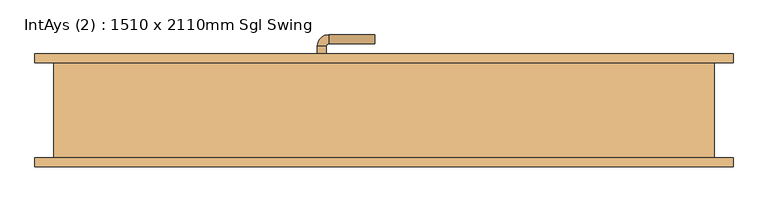
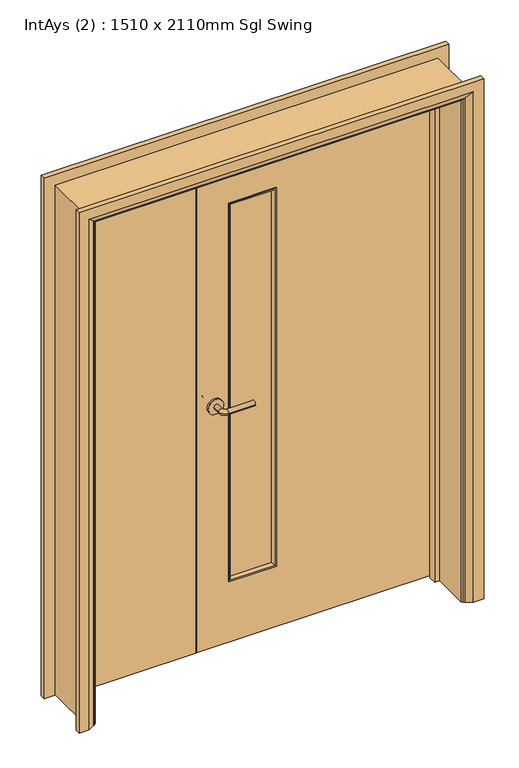
"""IFC4 building model written with IfcOpenShell, lengths in millimetres: door geometry, IntAys (2) : 1510 x 2110mm Sgl Swing."""

from ifc_helpers import new_model, si_unit, point, frame, frame_2d, origin, place, context, project, spatial, polyline, circle_curve, ellipse_curve, trimmed, segment, composite_curve, outline, extrude, faceted_brep, source, transform, mapped, element, save
from ifc_brep_helpers import plane_surface, cylinder_surface, revolved_surface, advanced_brep


def intays_2_1510_x_2110mm_sgl_swing_d010f506(model_context):
    return source(origin(), model_context, "Body", "SolidModel", [
        advanced_brep(
        [(88.5, 67.5, 1000.0), (108.5, 67.5, 1000.0), (108.5, 37.5, 1000.0), (88.5, 37.5, 1000.0), (113.5, 32.5, 1000.0), (113.5, 12.5, 1000.0), (218.5, 12.5, 1000.0), (218.5, 32.5, 1000.0)],
        [
            (0, 1, circle_curve(frame((98.5, 67.5, 1000.0), z_axis=(0.0, 1.0, 0.0), x_axis=(1.0, 0.0, 0.0)), 10.0)),
            (1, 0, circle_curve(frame((98.5, 67.5, 1000.0), z_axis=(0.0, 1.0, 0.0), x_axis=(1.0, 0.0, 0.0)), 10.0)),
            (1, 2),
            (2, 3, circle_curve(frame((98.5, 37.5, 1000.0), z_axis=(0.0, 1.0, 0.0), x_axis=(1.0, 0.0, 0.0)), 10.0)),
            (3, 0),
            (3, 2, circle_curve(frame((98.5, 37.5, 1000.0), z_axis=(0.0, 1.0, 0.0), x_axis=(1.0, 0.0, 0.0)), 10.0)),
            (4, 5, circle_curve(frame((113.5, 22.5, 1000.0), z_axis=(-1.0, 0.0, 0.0), x_axis=(0.0, 1.0, 0.0)), 10.0)),
            (5, 3, circle_curve(frame((113.5, 37.5, 1000.0), z_axis=(0.0, 0.0, -1.0), x_axis=(-1.0, 0.0, 0.0)), 25.0)),
            (2, 4, circle_curve(frame((113.5, 37.5, 1000.0), z_axis=(0.0, 0.0, 1.0), x_axis=(-1.0, 0.0, 0.0)), 5.0)),
            (5, 4, circle_curve(frame((113.5, 22.5, 1000.0), z_axis=(-1.0, 0.0, 0.0), x_axis=(0.0, 1.0, 0.0)), 10.0)),
            (6, 7, circle_curve(frame((218.5, 22.5, 1000.0), z_axis=(1.0, 0.0, 0.0), x_axis=(0.0, 1.0, 0.0)), 10.0)),
            (7, 6, circle_curve(frame((218.5, 22.5, 1000.0), z_axis=(1.0, 0.0, 0.0), x_axis=(0.0, 1.0, 0.0)), 10.0)),
            (4, 7),
            (6, 5),
        ],
        [
            plane_surface(frame((98.5, 67.5, 1000.0), z_axis=(0.0, 1.0, 0.0), x_axis=(0.0, 0.0, 1.0))),
            cylinder_surface(frame((98.5, 67.5, 1000.0), z_axis=(0.0, 1.0, 0.0), x_axis=(1.0, 0.0, 0.0)), 10.0),
            revolved_surface(trimmed(ellipse_curve(frame((98.5, 37.5, 1000.0), z_axis=(0.0, -1.0, 0.0), x_axis=(1.0, 0.0, 0.0)), 10.0, 10.0), [point((88.5, 37.5, 1000.0))], [point((108.5, 37.5, 1000.0))], True, "CARTESIAN"), (113.5, 37.5, 1000.0), (0.0, 0.0, -1.0)),
            revolved_surface(trimmed(ellipse_curve(frame((98.5, 37.5, 1000.0), z_axis=(0.0, -1.0, 0.0), x_axis=(1.0, 0.0, 0.0)), 10.0, 10.0), [point((108.5, 37.5, 1000.0))], [point((88.5, 37.5, 1000.0))], True, "CARTESIAN"), (113.5, 37.5, 1000.0), (0.0, 0.0, -1.0)),
            plane_surface(frame((218.5, 22.5, 1000.0), z_axis=(1.0, 0.0, 0.0), x_axis=(0.0, 0.0, 1.0))),
            cylinder_surface(frame((113.5, 22.5, 1000.0), z_axis=(-1.0, 0.0, 0.0), x_axis=(0.0, 1.0, 0.0)), 10.0),
        ],
        [
            (0, [[1, 2]]),
            (1, [[3, 4, 5, -2]]),
            (1, [[-5, 6, -3, -1]]),
            (2, [[7, 8, -4, 9]]),
            (3, [[10, -9, -6, -8]]),
            (4, [[11, 12]]),
            (5, [[13, -11, 14, -7]]),
            (5, [[-14, -12, -13, -10]]),
        ],
    ),
        extrude(outline(composite_curve([segment(trimmed(circle_curve(frame_2d((1000.0, 96.0)), 30.0), [point((1000.0, 66.0))], [point((1000.0, 126.0))], False, "CARTESIAN"), True, "CONTINUOUS"), segment(trimmed(circle_curve(frame_2d((1000.0, 96.0)), 30.0), [point((1000.0, 126.0))], [point((1000.0, 66.0))], False, "CARTESIAN"), True, "CONTINUOUS")], self_intersect=False)), frame((0.0, 67.5, 0.0), z_axis=(0.0, 1.0, 0.0), x_axis=(0.0, 0.0, 1.0)), (0.0, 0.0, 1.0), 8.0),
        advanced_brep(
        [(88.5, 115.5, 1000.0), (108.5, 115.5, 1000.0), (88.5, 145.5, 1000.0), (108.5, 145.5, 1000.0), (113.5, 150.5, 1000.0), (113.5, 170.5, 1000.0), (218.5, 170.5, 1000.0), (218.5, 150.5, 1000.0)],
        [
            (0, 1, circle_curve(frame((98.5, 115.5, 1000.0), z_axis=(0.0, -1.0, 0.0), x_axis=(1.0, 0.0, 0.0)), 10.0)),
            (1, 0, circle_curve(frame((98.5, 115.5, 1000.0), z_axis=(0.0, -1.0, 0.0), x_axis=(1.0, 0.0, 0.0)), 10.0)),
            (0, 2),
            (2, 3, circle_curve(frame((98.5, 145.5, 1000.0), z_axis=(0.0, -1.0, 0.0), x_axis=(1.0, 0.0, 0.0)), 10.0)),
            (3, 1),
            (3, 2, circle_curve(frame((98.5, 145.5, 1000.0), z_axis=(0.0, -1.0, 0.0), x_axis=(1.0, 0.0, 0.0)), 10.0)),
            (4, 3, circle_curve(frame((113.5, 145.5, 1000.0), z_axis=(0.0, 0.0, 1.0), x_axis=(-1.0, 0.0, 0.0)), 5.0)),
            (2, 5, circle_curve(frame((113.5, 145.5, 1000.0), z_axis=(0.0, 0.0, -1.0), x_axis=(-1.0, 0.0, 0.0)), 25.0)),
            (5, 4, circle_curve(frame((113.5, 160.5, 1000.0), z_axis=(-1.0, 0.0, 0.0), x_axis=(0.0, -1.0, 0.0)), 10.0)),
            (4, 5, circle_curve(frame((113.5, 160.5, 1000.0), z_axis=(-1.0, 0.0, 0.0), x_axis=(0.0, -1.0, 0.0)), 10.0)),
            (6, 7, circle_curve(frame((218.5, 160.5, 1000.0), z_axis=(1.0, 0.0, 0.0), x_axis=(0.0, -1.0, 0.0)), 10.0)),
            (7, 6, circle_curve(frame((218.5, 160.5, 1000.0), z_axis=(1.0, 0.0, 0.0), x_axis=(0.0, -1.0, 0.0)), 10.0)),
            (5, 6),
            (7, 4),
        ],
        [
            plane_surface(frame((98.5, 115.5, 1000.0), z_axis=(0.0, -1.0, 0.0), x_axis=(0.0, 0.0, 1.0))),
            cylinder_surface(frame((98.5, 115.5, 1000.0), z_axis=(0.0, -1.0, 0.0), x_axis=(1.0, 0.0, 0.0)), 10.0),
            revolved_surface(trimmed(ellipse_curve(frame((98.5, 145.5, 1000.0), z_axis=(0.0, -1.0, 0.0), x_axis=(1.0, 0.0, 0.0)), 10.0, 10.0), [point((88.5, 145.5, 1000.0))], [point((108.5, 145.5, 1000.0))], True, "CARTESIAN"), (113.5, 145.5, 1000.0), (0.0, 0.0, -1.0)),
            revolved_surface(trimmed(ellipse_curve(frame((98.5, 145.5, 1000.0), z_axis=(0.0, -1.0, 0.0), x_axis=(1.0, 0.0, 0.0)), 10.0, 10.0), [point((108.5, 145.5, 1000.0))], [point((88.5, 145.5, 1000.0))], True, "CARTESIAN"), (113.5, 145.5, 1000.0), (0.0, 0.0, -1.0)),
            plane_surface(frame((218.5, 160.5, 1000.0), z_axis=(1.0, 0.0, 0.0), x_axis=(0.0, 0.0, 1.0))),
            cylinder_surface(frame((113.5, 160.5, 1000.0), z_axis=(-1.0, 0.0, 0.0), x_axis=(0.0, -1.0, 0.0)), 10.0),
        ],
        [
            (0, [[1, 2]]),
            (1, [[-1, 3, 4, 5]]),
            (1, [[-2, -5, 6, -3]]),
            (2, [[7, -4, 8, 9]]),
            (3, [[-8, -6, -7, 10]]),
            (4, [[11, 12]]),
            (5, [[-9, 13, -12, 14]]),
            (5, [[-10, -14, -11, -13]]),
        ],
    ),
        extrude(outline(composite_curve([segment(trimmed(circle_curve(frame_2d((1000.0, 96.0)), 30.0), [point((1000.0, 66.0))], [point((1000.0, 126.0))], False, "CARTESIAN"), True, "CONTINUOUS"), segment(trimmed(circle_curve(frame_2d((1000.0, 96.0)), 30.0), [point((1000.0, 126.0))], [point((1000.0, 66.0))], False, "CARTESIAN"), True, "CONTINUOUS")], self_intersect=False)), frame((0.0, 107.5, 0.0), z_axis=(0.0, 1.0, 0.0), x_axis=(0.0, 0.0, 1.0)), (0.0, 0.0, 1.0), 8.0),
        extrude(outline(polyline([(2102.0, -508.0), (0.0, -508.0), (0.0, -476.0), (2070.0, -476.0), (2070.0, 954.0), (0.0, 954.0), (0.0, 986.0), (2102.0, 986.0), (2102.0, -508.0)])), frame((0.0, -107.5, 0.0), z_axis=(0.0, 1.0, 0.0), x_axis=(0.0, 0.0, 1.0)), (0.0, 0.0, 1.0), 215.0),
        advanced_brep(
        [(-551.0, -127.5, 0.0), (-551.0, -107.5, 0.0), (-481.0, -107.5, 0.0), (-485.0, -113.5, 0.0), (-511.0, -127.5, 0.0), (-551.0, -127.5, 2145.0), (-551.0, -107.5, 2145.0), (1029.0, -107.5, 2145.0), (1029.0, -107.5, 0.0), (959.0, -107.5, 0.0), (959.0, -107.5, 2075.0), (-481.0, -107.5, 2075.0), (-485.0, -113.5, 2079.0), (-511.0, -127.5, 2105.0), (989.0, -127.5, 2105.0), (989.0, -127.5, 0.0), (1029.0, -127.5, 0.0), (1029.0, -127.5, 2145.0), (963.0, -113.5, 0.0), (963.0, -113.5, 2079.0)],
        [
            (0, 1),
            (1, 2),
            (2, 3, circle_curve(frame((-489.0, -106.5, 0.0), z_axis=(0.0, 0.0, -1.0), x_axis=(-1.0, 0.0, 0.0)), 8.0622577)),
            (3, 4),
            (4, 0),
            (0, 5),
            (5, 6),
            (6, 1),
            (6, 7),
            (7, 8),
            (8, 9),
            (9, 10),
            (10, 11),
            (11, 2),
            (11, 12, ellipse_curve(frame((-489.0, -106.5, 2083.0), z_axis=(-0.7071067811865475, 0.0, -0.7071067811865475), x_axis=(0.7071067811865474, 0.0, -0.7071067811865476)), 11.4017543, 8.0622577)),
            (12, 3),
            (12, 13),
            (13, 4),
            (13, 14),
            (14, 15),
            (15, 16),
            (16, 17),
            (17, 5),
            (7, 17),
            (16, 8),
            (15, 18),
            (18, 9, circle_curve(frame((967.0, -106.5, 0.0), z_axis=(0.0, 0.0, -1.0), x_axis=(1.0, 0.0, 0.0)), 8.0622577)),
            (19, 10, ellipse_curve(frame((967.0, -106.5, 2083.0), z_axis=(0.7071067811865475, 0.0, -0.7071067811865475), x_axis=(0.7071067811865474, 0.0, 0.7071067811865476)), 11.4017543, 8.0622577)),
            (18, 19),
            (14, 19),
            (19, 12),
        ],
        [
            plane_surface(frame((-481.0, -107.5, 0.0), z_axis=(0.0, 0.0, -1.0), x_axis=(0.0, -1.0, 0.0))),
            plane_surface(frame((-551.0, -127.5, 0.0), z_axis=(-1.0, 0.0, 0.0), x_axis=(0.0, 0.0, 1.0))),
            plane_surface(frame((-551.0, -107.5, 0.0), z_axis=(0.0, 1.0, 0.0), x_axis=(0.0, 0.0, 1.0))),
            cylinder_surface(frame((-489.0, -106.5, 0.0), z_axis=(0.0, 0.0, -1.0), x_axis=(-1.0, 0.0, 0.0)), 8.0622577),
            plane_surface(frame((-485.0, -113.5, 0.0), z_axis=(0.4740998230350183, -0.8804710999221749, 0.0), x_axis=(0.0, 0.0, 1.0))),
            plane_surface(frame((-511.0, -127.5, 0.0), z_axis=(0.0, -1.0, 0.0), x_axis=(0.0, 0.0, 1.0))),
            plane_surface(frame((1029.0, -127.5, 2145.0), z_axis=(1.0, 0.0, 0.0), x_axis=(0.0, 0.0, -1.0))),
            plane_surface(frame((959.0, -107.5, 0.0), z_axis=(0.0, 0.0, -1.0), x_axis=(0.0, -1.0, 0.0))),
            cylinder_surface(frame((967.0, -106.5, 2075.0), z_axis=(0.0, 0.0, 1.0), x_axis=(1.0, 0.0, 0.0)), 8.0622577),
            plane_surface(frame((963.0, -113.5, 2079.0), z_axis=(-0.4740998230350183, -0.8804710999221749, 0.0), x_axis=(0.0, 0.0, -1.0))),
            plane_surface(frame((-551.0, -127.5, 2145.0), z_axis=(0.0, 0.0, 1.0), x_axis=(1.0, 0.0, 0.0))),
            cylinder_surface(frame((-481.0, -106.5, 2083.0), z_axis=(-1.0, 0.0, 0.0), x_axis=(0.0, 0.0, 1.0)), 8.0622577),
            plane_surface(frame((-485.0, -113.5, 2079.0), z_axis=(0.0, -0.8804710999221749, -0.4740998230350183), x_axis=(1.0, 0.0, 0.0))),
        ],
        [
            (0, [[1, 2, 3, 4, 5]]),
            (1, [[-1, 6, 7, 8]]),
            (2, [[-2, -8, 9, 10, 11, 12, 13, 14]]),
            (3, [[-3, -14, 15, 16]]),
            (4, [[-4, -16, 17, 18]]),
            (5, [[-5, -18, 19, 20, 21, 22, 23, -6]]),
            (6, [[24, -22, 25, -10]]),
            (7, [[-21, 26, 27, -11, -25]]),
            (8, [[28, -12, -27, 29]]),
            (9, [[30, -29, -26, -20]]),
            (10, [[-7, -23, -24, -9]]),
            (11, [[-15, -13, -28, 31]]),
            (12, [[-17, -31, -30, -19]]),
        ],
    ),
        advanced_brep(
        [(1029.0, 127.5, 0.0), (1029.0, 107.5, 0.0), (959.0, 107.5, 0.0), (963.0, 113.5, 0.0), (989.0, 127.5, 0.0), (1029.0, 127.5, 2145.0), (1029.0, 107.5, 2145.0), (-551.0, 107.5, 2145.0), (-551.0, 107.5, 0.0), (-481.0, 107.5, 0.0), (-481.0, 107.5, 2075.0), (959.0, 107.5, 2075.0), (963.0, 113.5, 2079.0), (989.0, 127.5, 2105.0), (-511.0, 127.5, 2105.0), (-511.0, 127.5, 0.0), (-551.0, 127.5, 0.0), (-551.0, 127.5, 2145.0), (-485.0, 113.5, 0.0), (-485.0, 113.5, 2079.0)],
        [
            (0, 1),
            (1, 2),
            (2, 3, circle_curve(frame((967.0, 106.5, 0.0), z_axis=(0.0, 0.0, -1.0), x_axis=(1.0, 0.0, 0.0)), 8.0622577)),
            (3, 4),
            (4, 0),
            (0, 5),
            (5, 6),
            (6, 1),
            (6, 7),
            (7, 8),
            (8, 9),
            (9, 10),
            (10, 11),
            (11, 2),
            (11, 12, ellipse_curve(frame((967.0, 106.5, 2083.0), z_axis=(0.7071067811865475, 0.0, -0.7071067811865475), x_axis=(-0.7071067811865474, 0.0, -0.7071067811865476)), 11.4017543, 8.0622577)),
            (12, 3),
            (12, 13),
            (13, 4),
            (13, 14),
            (14, 15),
            (15, 16),
            (16, 17),
            (17, 5),
            (7, 17),
            (16, 8),
            (15, 18),
            (18, 9, circle_curve(frame((-489.0, 106.5, 0.0), z_axis=(0.0, 0.0, -1.0), x_axis=(-1.0, 0.0, 0.0)), 8.0622577)),
            (19, 10, ellipse_curve(frame((-489.0, 106.5, 2083.0), z_axis=(-0.7071067811865475, 0.0, -0.7071067811865475), x_axis=(-0.7071067811865474, 0.0, 0.7071067811865476)), 11.4017543, 8.0622577)),
            (18, 19),
            (14, 19),
            (19, 12),
        ],
        [
            plane_surface(frame((959.0, 107.5, 0.0), z_axis=(0.0, 0.0, -1.0), x_axis=(0.0, -1.0, 0.0))),
            plane_surface(frame((1029.0, 127.5, 0.0), z_axis=(1.0, 0.0, 0.0), x_axis=(0.0, 0.0, 1.0))),
            plane_surface(frame((1029.0, 107.5, 0.0), z_axis=(0.0, -1.0, 0.0), x_axis=(0.0, 0.0, 1.0))),
            cylinder_surface(frame((967.0, 106.5, 0.0), z_axis=(0.0, 0.0, -1.0), x_axis=(1.0, 0.0, 0.0)), 8.0622577),
            plane_surface(frame((963.0, 113.5, 0.0), z_axis=(-0.4740998230350126, 0.8804710999221779, 0.0), x_axis=(0.0, 0.0, 1.0))),
            plane_surface(frame((989.0, 127.5, 0.0), z_axis=(0.0, 1.0, 0.0), x_axis=(0.0, 0.0, 1.0))),
            plane_surface(frame((-551.0, 127.5, 2145.0), z_axis=(-1.0, 0.0, 0.0), x_axis=(0.0, 0.0, -1.0))),
            plane_surface(frame((-481.0, 107.5, 0.0), z_axis=(0.0, 0.0, -1.0), x_axis=(0.0, -1.0, 0.0))),
            cylinder_surface(frame((-489.0, 106.5, 2075.0), z_axis=(0.0, 0.0, 1.0), x_axis=(-1.0, 0.0, 0.0)), 8.0622577),
            plane_surface(frame((-485.0, 113.5, 2079.0), z_axis=(0.4740998230350183, 0.8804710999221749, 0.0), x_axis=(0.0, 0.0, -1.0))),
            plane_surface(frame((1029.0, 127.5, 2145.0), z_axis=(0.0, 0.0, 1.0), x_axis=(-1.0, 0.0, 0.0))),
            cylinder_surface(frame((959.0, 106.5, 2083.0), z_axis=(1.0, 0.0, 0.0), x_axis=(0.0, 0.0, 1.0)), 8.0622577),
            plane_surface(frame((963.0, 113.5, 2079.0), z_axis=(0.0, 0.8804710999221763, -0.4740998230350154), x_axis=(-1.0, 0.0, 0.0))),
        ],
        [
            (0, [[1, 2, 3, 4, 5]]),
            (1, [[-1, 6, 7, 8]]),
            (2, [[-2, -8, 9, 10, 11, 12, 13, 14]]),
            (3, [[-3, -14, 15, 16]]),
            (4, [[-4, -16, 17, 18]]),
            (5, [[-5, -18, 19, 20, 21, 22, 23, -6]]),
            (6, [[24, -22, 25, -10]]),
            (7, [[-21, 26, 27, -11, -25]]),
            (8, [[28, -12, -27, 29]]),
            (9, [[30, -29, -26, -20]]),
            (10, [[-7, -23, -24, -9]]),
            (11, [[-15, -13, -28, 31]]),
            (12, [[-17, -31, -30, -19]]),
        ],
    ),
        faceted_brep([(-457.0, 72.5, 0.0), (-457.0, 40.5, 0.0), (-476.0, 40.5, 0.0), (-476.0, 72.5, 0.0), (-457.0, 72.5, 2051.0), (-457.0, 40.5, 2051.0), (-476.0, 40.5, 2070.0), (-476.0, 72.5, 2070.0), (935.0, 72.5, 0.0), (954.0, 72.5, 0.0), (954.0, 40.5, 0.0), (935.0, 40.5, 0.0), (935.0, 72.5, 2051.0), (954.0, 72.5, 2070.0), (954.0, 40.5, 2070.0), (935.0, 40.5, 2051.0)], [[[0, 1, 2, 3]], [[1, 0, 4, 5]], [[2, 1, 5, 6]], [[3, 2, 6, 7]], [[0, 3, 7, 4]], [[8, 9, 10, 11]], [[12, 13, 9, 8]], [[13, 14, 10, 9]], [[14, 15, 11, 10]], [[15, 12, 8, 11]], [[5, 4, 12, 15]], [[6, 5, 15, 14]], [[7, 6, 14, 13]], [[4, 7, 13, 12]]]),
        extrude(outline(polyline([(335.0, 85.5), (150.0, 85.5), (150.0, 97.5), (335.0, 97.5), (335.0, 85.5)])), frame((0.0, 0.0, 257.0), z_axis=(0.0, 0.0, 1.0), x_axis=(1.0, 0.0, 0.0)), (0.0, 0.0, 1.0), 1560.0),
        extrude(outline(polyline([(22.0, 75.5), (-473.0, 75.5), (-473.0, 107.5), (22.0, 107.5), (22.0, 75.5)])), frame((0.0, 0.0, 5.753223), z_axis=(0.0, 0.0, 1.0), x_axis=(1.0, 0.0, 0.0)), (0.0, 0.0, 1.0), 2061.246777),
        extrude(outline(polyline([(5.753223, 951.0), (2067.0, 951.0), (2067.0, 25.0), (5.753223, 25.0), (5.753223, 951.0)]), holes=[polyline([(1817.0, 150.0), (1817.0, 335.0), (257.0, 335.0), (257.0, 150.0), (1817.0, 150.0)])]), frame((0.0, 75.5, 0.0), z_axis=(0.0, 1.0, 0.0), x_axis=(0.0, 0.0, 1.0)), (0.0, 0.0, 1.0), 32.0),
        faceted_brep([(335.0, 72.5, 257.0), (335.0, 85.5, 257.0), (335.0, 85.5, 1817.0), (335.0, 72.5, 1817.0), (323.0, 85.5, 269.0), (329.0, 72.5, 263.0), (329.0, 72.5, 1811.0), (323.0, 85.5, 1805.0), (150.0, 85.5, 1817.0), (150.0, 72.5, 1817.0), (156.0, 72.5, 1811.0), (162.0, 85.5, 1805.0), (150.0, 85.5, 257.0), (150.0, 72.5, 257.0), (156.0, 72.5, 263.0), (162.0, 85.5, 269.0)], [[[0, 1, 2, 3]], [[4, 5, 6, 7]], [[3, 2, 8, 9]], [[7, 6, 10, 11]], [[9, 8, 12, 13]], [[11, 10, 14, 15]], [[1, 12, 8, 2], [7, 11, 15, 4]], [[13, 12, 1, 0]], [[3, 9, 13, 0], [5, 14, 10, 6]], [[15, 14, 5, 4]]]),
        faceted_brep([(150.0, 110.5, 257.0), (150.0, 97.5, 257.0), (150.0, 97.5, 1817.0), (150.0, 110.5, 1817.0), (162.0, 97.5, 269.0), (156.0, 110.5, 263.0), (156.0, 110.5, 1811.0), (162.0, 97.5, 1805.0), (335.0, 97.5, 1817.0), (335.0, 110.5, 1817.0), (329.0, 110.5, 1811.0), (323.0, 97.5, 1805.0), (335.0, 97.5, 257.0), (335.0, 110.5, 257.0), (329.0, 110.5, 263.0), (323.0, 97.5, 269.0)], [[[0, 1, 2, 3]], [[4, 5, 6, 7]], [[3, 2, 8, 9]], [[7, 6, 10, 11]], [[9, 8, 12, 13]], [[11, 10, 14, 15]], [[1, 12, 8, 2], [7, 11, 15, 4]], [[13, 12, 1, 0]], [[3, 9, 13, 0], [5, 14, 10, 6]], [[15, 14, 5, 4]]]),
    ])


if __name__ == "__main__":
    model = new_model("IFC4")
    model_context = context("Model", 3, world=origin())
    ifc_project = project(units=[si_unit("LENGTHUNIT", "METRE", prefix="MILLI")], contexts=[model_context])
    site = spatial("IfcSite", under=ifc_project)
    building = spatial("IfcBuilding", under=site)
    placement = place(None, origin())
    intays_2_1510_x_2110mm_sgl_swing_shape = intays_2_1510_x_2110mm_sgl_swing_d010f506(model_context)
    element("IfcDoor", 1, ObjectType="IntAys (2) : 1510 x 2110mm Sgl Swing", at=placement, inside=building, context=model_context, shape_type="MappedRepresentation", body=[
        mapped(intays_2_1510_x_2110mm_sgl_swing_shape, transform((0.0, 0.0, 0.0), x_axis=(1.0, 0.0, 0.0), y_axis=(0.0, 1.0, 0.0), z_axis=(0.0, 0.0, 1.0))),
    ])
    save(model, "model.ifc")

# Revit data of these elements
# Type "IntAys (2) : 1510 x 2110mm Sgl Swing"
#   Type Mark = "46"
#   Type Comments = "Internal Asymmetric"
#   Operation = "DoubleDoorSingleSwing"
#   Construction Type Id = "SGL"
#   Keynote = "L20"
#   Description = "Internal Asymmetric Door"
#   Analytic Construction = "Large single-glazed windows"
#   Visual Light Transmittance = 0.9
#   VisionPanel Width = 185 mm
#   Thickness = 32 mm
#   Stop Thickness = 19 mm
#   Stop Depth = 32 mm
#   Stile Top Rail = 250 mm
#   Stile Shutting = 125 mm
#   Stile Bottom Rail = 250 mm
#   Solar Heat Gain Coefficient = 0.86
#   Secondary Panel Width = 495 mm
#   Rough Width = 1510 mm
#   Rough Height = 2110 mm
#   Main Panel Width = 926 mm
#   Heat Transfer Coefficient (U) = 5.5617 W/(m²·K)
#   Handle Z Distance = 1000 mm
#   Handle X Distance = 75 mm
#   Handle Length = 350 mm
#   Frame Thickness = 32 mm
#   Door Panel Width = 926 mm
#   Door Panel Thickness = 32 mm
#   Height = 2110 mm
#   Door Panel Offset = 0 mm
#   Structural Tolerance = 8 mm
#   Tolerance = 3 mm
#   UnderCut = 7 mm
#   Width = 1510 mm
#   Door Panel Height = 2060 mm
#   Architrave Setback = 5 mm
#   Vis - Swing Single = yes
#   Vis - Swing Opposing = no
#   Vis - Swing Double = no
#   Vis - Stops = yes
#   Vis - Ironmongery = yes
#   Define Thermal Properties by = 1
#   Material Ironmongery = Door - Handle
#   Material Glass = Door - Glazing
#   Material Frame = Door - Frame/Mullion
#   Material Door = Door - Panel
#   Material Beading = Door - Panel
#   Material Architrave = Door - Architrave
#   Handle Style = element 261135
#   Function = (empty or 0)
#   Wall Closure = (empty or 0)
# Element 1 (IfcDoor, "IntAys (2) : 1510 x 2110mm Sgl Swing")
#   Materials on its faces: "Door - Panel", "Door - Architrave", "Door - Handle", "Door - Frame/Mullion", "Door - Glazing"
# Materials
#   "Door - Handle": class "Miscellaneous", colour RGB 0 0 0, transparency 0, Keynote = "P21"
#   "Door - Glazing": class "Miscellaneous", colour RGB 0 0 255, transparency 0.75
#   "Door - Frame/Mullion": class "Wood", colour RGB 212 179 113, transparency 0, Keynote = "L20"
#   "Door - Panel": class "Wood", colour RGB 210 159 95, transparency 0, Keynote = "L20"
#   "Door - Architrave": class "Wood", colour RGB 154 90 5, transparency 0, Keynote = "P20"
